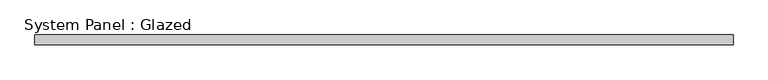
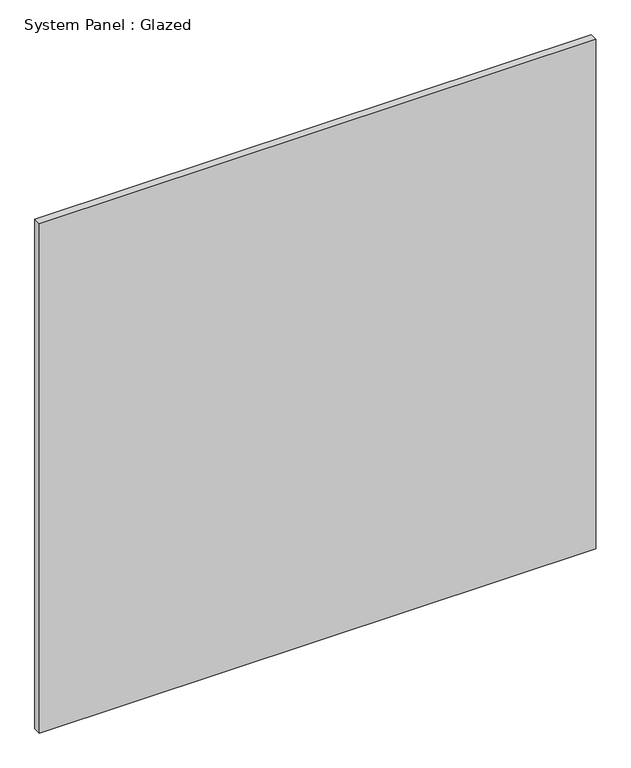
"""IFC4 building model written with IfcOpenShell, lengths in millimetres: plate geometry, System Panel : Glazed."""

from ifc_helpers import new_model, si_unit, origin, origin_with_axes, place, context, project, spatial, polyline, outline, extrude, source, transform, mapped, element, save


def system_panel_glazed_bac2966e(model_context):
    return source(origin(), model_context, "Body", "SweptSolid", [
        extrude(outline(polyline([(890.0, 24.5), (-890.0, 24.5), (-890.0, 49.5), (890.0, 49.5), (890.0, 24.5)])), origin_with_axes(), (0.0, 0.0, 1.0), 1722.3836314),
    ])


if __name__ == "__main__":
    model = new_model("IFC4")
    model_context = context("Model", 3, world=origin())
    ifc_project = project(units=[si_unit("LENGTHUNIT", "METRE", prefix="MILLI")], contexts=[model_context])
    site = spatial("IfcSite", under=ifc_project)
    building = spatial("IfcBuilding", under=site)
    placement = place(None, origin())
    system_panel_glazed_shape = system_panel_glazed_bac2966e(model_context)
    element("IfcPlate", 1, ObjectType="System Panel : Glazed", at=placement, inside=building, context=model_context, shape_type="MappedRepresentation", body=[
        mapped(system_panel_glazed_shape, transform((0.0, 0.0, 0.0), x_axis=(1.0, 0.0, 0.0), y_axis=(0.0, 1.0, 0.0), z_axis=(0.0, 0.0, 1.0))),
    ])
    save(model, "model.ifc")

# Revit data of these elements
# Element 1 (IfcPlate, "System Panel : Glazed")
#   Materials on its faces: "Glass"
# Materials
#   "Glass": class "Glass", colour RGB 218 227 224, transparency 0.85, Description = "Soda Lime Glass", Cost = 0
